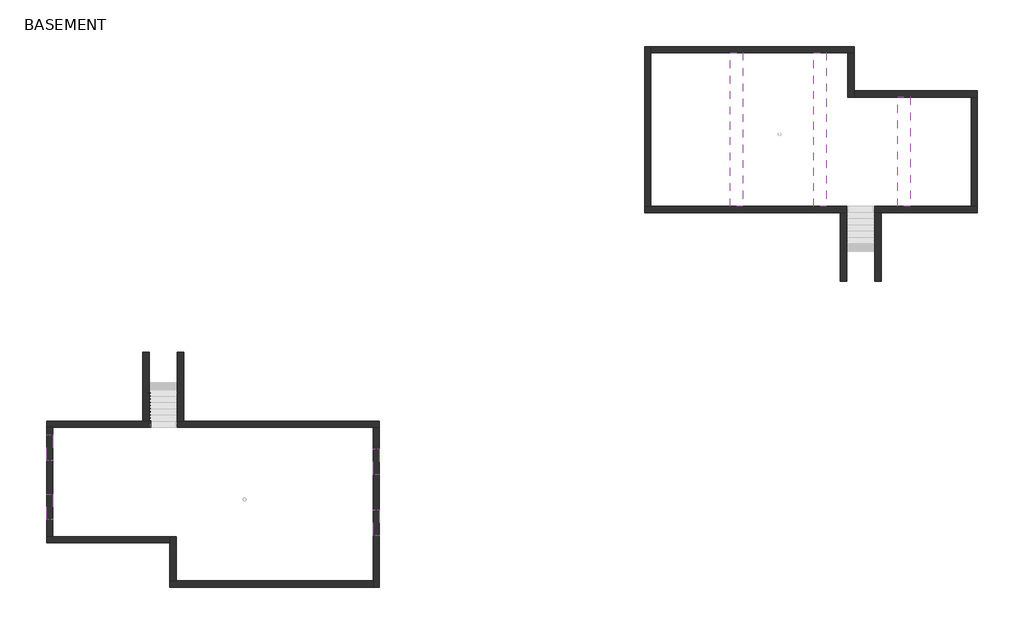
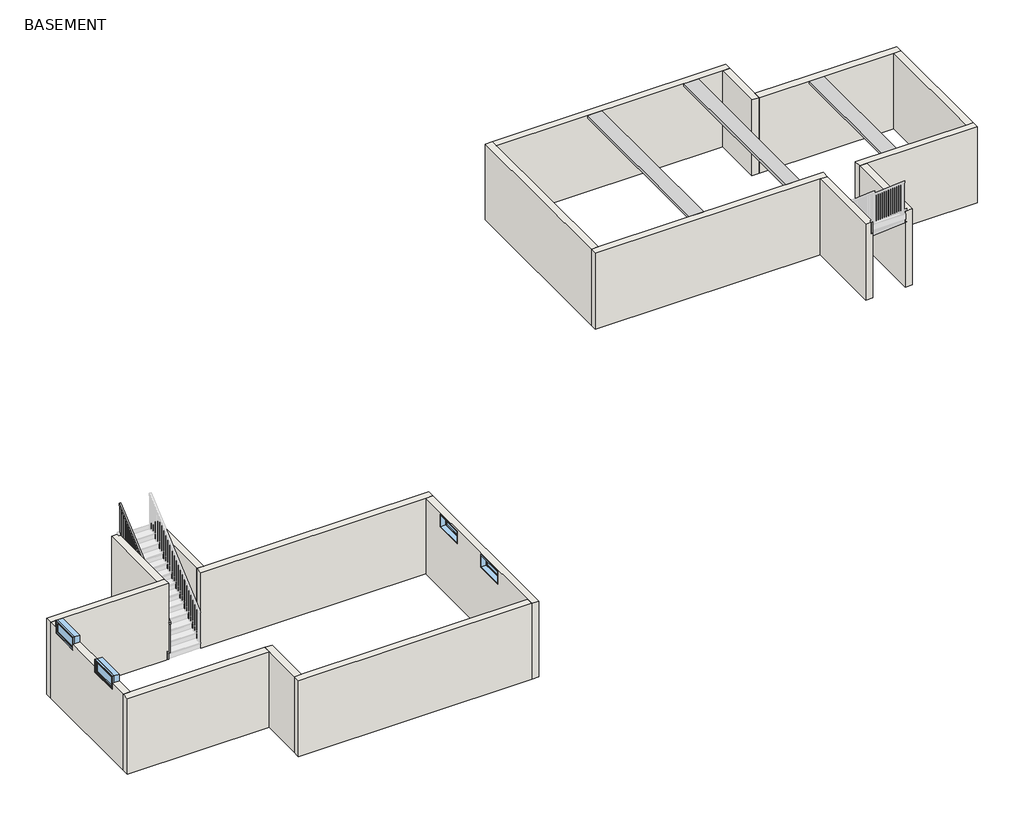
# One storey, part 1 of 2: 18 walls, 4 windows, 3 beams, 1 railing.
"""IFC4 building model written with IfcOpenShell, lengths in millimetres."""

import ifcopenshell
import ifcopenshell.guid

model = None  # the IFC model being written
_history = None  # IfcOwnerHistory: only IFC2X3 demands one
_inside = {}  # id of a spatial element -> (the spatial element, [elements in it])
_under = {}  # id of a project, library or spatial element -> (it, [spatial elements below it])
_declared = {}  # id of a project -> (the project, [libraries it declares])
_typed = {}  # id of a type object -> (the type object, [elements of that type])
_made_of = {}  # id of a material, layer set ... -> (it, [elements and type objects made of it])


def new_model(schema):
    """Start an empty IFC model of exactly this schema.

    Asked for "IFC4X3", IfcOpenShell would pick the latest addendum, in which some entities
    have other attributes; the version numbers below select the first issue.
    IFC2X3 requires an IfcOwnerHistory on every rooted entity: one is made here for all.
    """
    global model, _history
    if schema == "IFC4X3":
        model = ifcopenshell.file(schema_version=(4, 3, 0, 0))
    else:
        model = ifcopenshell.file(schema=schema)
    _inside.clear()
    _under.clear()
    _declared.clear()
    _typed.clear()
    _made_of.clear()
    _history = None
    if model.schema == "IFC2X3":
        org = make("IfcOrganization", Name="unknown")
        user = make(
            "IfcPersonAndOrganization",
            ThePerson=make("IfcPerson", FamilyName="unknown"),
            TheOrganization=org,
        )
        app = make(
            "IfcApplication",
            ApplicationDeveloper=org,
            Version="unknown",
            ApplicationFullName="unknown",
            ApplicationIdentifier="unknown",
        )
        _history = make(
            "IfcOwnerHistory",
            OwningUser=user,
            OwningApplication=app,
            ChangeAction="ADDED",
            CreationDate=0,
        )
    return model


def make(cls, **values):
    """One entity of the class cls with the attributes given. An attribute that is None is left unset."""
    return model.create_entity(
        cls, **{name: value for name, value in values.items() if value is not None}
    )


def rooted(cls, **values):
    """An entity with a GlobalId (a new one), such as an element, a storey or a relation."""
    return make(cls, GlobalId=ifcopenshell.guid.new(), OwnerHistory=_history, **values)


def si_unit(unit_type, name, prefix=None):
    """IfcSIUnit, for example si_unit("LENGTHUNIT", "METRE", prefix="MILLI")."""
    return make("IfcSIUnit", UnitType=unit_type, Prefix=prefix, Name=name)


def assignment(units):
    """IfcUnitAssignment: the units of a project."""
    return None if units is None else make("IfcUnitAssignment", Units=units)


def point(xyz):
    """IfcCartesianPoint."""
    return None if xyz is None else make("IfcCartesianPoint", Coordinates=xyz)


def direction(xyz):
    """IfcDirection."""
    return None if xyz is None else make("IfcDirection", DirectionRatios=xyz)


def frame(location, z_axis=None, x_axis=None):
    """IfcAxis2Placement3D, a coordinate frame: its origin and axes. An axis left out is left unset."""
    return make(
        "IfcAxis2Placement3D",
        Location=point(location),
        Axis=direction(z_axis),
        RefDirection=direction(x_axis),
    )


def origin():
    """The frame at (0, 0, 0) with its axes left unset."""
    return frame((0.0, 0.0, 0.0))


def place(relative_to, where):
    """IfcLocalPlacement: puts the frame where relative to a parent placement (None: the world)."""
    return make(
        "IfcLocalPlacement", PlacementRelTo=relative_to, RelativePlacement=where
    )


def context(
    kind, dimensions, precision=None, world=None, true_north=None, identifier=None
):
    """IfcGeometricRepresentationContext, for example the 3D "Model" context."""
    return make(
        "IfcGeometricRepresentationContext",
        ContextIdentifier=identifier,
        ContextType=kind,
        CoordinateSpaceDimension=dimensions,
        Precision=precision,
        WorldCoordinateSystem=world,
        TrueNorth=true_north,
    )


def project(units=None, contexts=None):
    """IfcProject with its units and contexts."""
    return rooted(
        "IfcProject",
        Name="project",
        RepresentationContexts=contexts,
        UnitsInContext=assignment(units),
    )


def spatial(cls, under=None, at=None, **own):
    """A site, building, storey or space (cls), placed at a placement, below another one or the project."""
    s = rooted(cls, ObjectPlacement=at, **own)
    if under is not None:
        _under.setdefault(under.id(), (under, []))[1].append(s)
    return s


def polyline(points):
    """IfcPolyline through the points."""
    return make("IfcPolyline", Points=[point(p) for p in points])


def outline(outer, holes=None, kind="AREA"):
    """IfcArbitraryClosedProfileDef: a profile drawn as a closed curve; with holes, ...WithVoids."""
    if holes is None:
        return make("IfcArbitraryClosedProfileDef", ProfileType=kind, OuterCurve=outer)
    return make(
        "IfcArbitraryProfileDefWithVoids",
        ProfileType=kind,
        OuterCurve=outer,
        InnerCurves=holes,
    )


def extrude(swept, where, along, depth):
    """IfcExtrudedAreaSolid: the profile swept, set in the frame where, extruded along a direction by depth."""
    return make(
        "IfcExtrudedAreaSolid",
        SweptArea=swept,
        Position=where,
        ExtrudedDirection=direction(along),
        Depth=depth,
    )


def faces_of(points, faces, orient=None, outer=None):
    """IfcFace entities. A face is a list of loops; a loop is a list of indices into points, from 0.

    orient and outer hold one flag for each loop. By default every Orientation is true, the
    first loop of a face is its IfcFaceOuterBound and the others are IfcFaceBound.
    """
    made = []
    for i, loops in enumerate(faces):
        bounds = []
        for j, loop in enumerate(loops):
            is_outer = j == 0 if outer is None else outer[i][j]
            bounds.append(
                make(
                    "IfcFaceOuterBound" if is_outer else "IfcFaceBound",
                    Bound=make("IfcPolyLoop", Polygon=[points[k] for k in loop]),
                    Orientation=True if orient is None else orient[i][j],
                )
            )
        made.append(make("IfcFace", Bounds=bounds))
    return made


def faceted_brep(points, faces, orient=None, outer=None, voids=None):
    """IfcFacetedBrep: a solid bounded by flat faces; with voids (closed shells), ...WithVoids."""
    shared = [point(p) for p in points]
    hull = make("IfcClosedShell", CfsFaces=faces_of(shared, faces, orient, outer))
    if voids is None:
        return make("IfcFacetedBrep", Outer=hull)
    return make(
        "IfcFacetedBrepWithVoids",
        Outer=hull,
        Voids=[
            make(cls, CfsFaces=faces_of(shared, fs, o, b)) for cls, fs, o, b in voids
        ],
    )


def shape(context_of_items, identifier, shape_type, items):
    """IfcShapeRepresentation: the items that make up one representation, for example the "Body"."""
    return make(
        "IfcShapeRepresentation",
        ContextOfItems=context_of_items,
        RepresentationIdentifier=identifier,
        RepresentationType=shape_type,
        Items=items,
    )


def source(mapping_origin, context_of_items, identifier, shape_type, items):
    """IfcRepresentationMap: a shape defined once, which mapped items show again and again."""
    return make(
        "IfcRepresentationMap",
        MappingOrigin=mapping_origin,
        MappedRepresentation=shape(context_of_items, identifier, shape_type, items),
    )


def transform(
    local_origin,
    x_axis=None,
    y_axis=None,
    z_axis=None,
    scale=None,
    scale2=None,
    scale3=None,
    uniform=True,
):
    """IfcCartesianTransformationOperator3D, or its non-uniform kind. x_axis, y_axis, z_axis: its Axis1, 2, 3."""
    if uniform:
        return make(
            "IfcCartesianTransformationOperator3D",
            Axis1=direction(x_axis),
            Axis2=direction(y_axis),
            LocalOrigin=point(local_origin),
            Scale=scale,
            Axis3=direction(z_axis),
        )
    return make(
        "IfcCartesianTransformationOperator3DnonUniform",
        Axis1=direction(x_axis),
        Axis2=direction(y_axis),
        LocalOrigin=point(local_origin),
        Scale=scale,
        Axis3=direction(z_axis),
        Scale2=scale2,
        Scale3=scale3,
    )


def mapped(mapping_source, mapping_target):
    """IfcMappedItem: shows the shape of a source again, moved by a transform."""
    return make(
        "IfcMappedItem", MappingSource=mapping_source, MappingTarget=mapping_target
    )


def made_of(thing, what):
    """Note that an element or type object is made of a material, layer set ...; save() writes the relation."""
    if what is not None:
        _made_of.setdefault(what.id(), (what, []))[1].append(thing)
    return thing


def element(
    cls,
    number,
    at=None,
    inside=None,
    cuts=None,
    type_object=None,
    material=None,
    context=None,
    identifier="Body",
    shape_type=None,
    held_by="IfcProductDefinitionShape",
    body=None,
    shapes=None,
    **own,
):
    """One element of the class cls, such as IfcWall. Its Tag is "e" and its number.

    at: its placement. inside: the storey or other place that contains it. cuts: it is an
    opening in that element (IfcRelVoidsElement). A single representation is given by context,
    identifier, shape_type and body (its items); several are given by shapes. held_by: the class
    of the entity that holds the representations. save() writes the other relations.
    """
    e = rooted(cls, Tag="e%d" % number, ObjectPlacement=at, **own)
    if body is not None:
        shapes = [shape(context, identifier, shape_type, body)]
    if shapes is not None:
        e.Representation = make(held_by, Representations=shapes)
    if inside is not None:
        _inside.setdefault(inside.id(), (inside, []))[1].append(e)
    if cuts is not None:
        rooted(
            "IfcRelVoidsElement", RelatingBuildingElement=cuts, RelatedOpeningElement=e
        )
    if type_object is not None:
        _typed.setdefault(type_object.id(), (type_object, []))[1].append(e)
    return made_of(e, material)


def aggregate(whole, parts):
    """IfcRelAggregates: a whole, such as a stair, and the parts it consists of."""
    return rooted("IfcRelAggregates", RelatingObject=whole, RelatedObjects=parts)


def save(model, path):
    """Write the relations noted so far, then the file.

    IfcRelAggregates (storeys below a building ...), IfcRelContainedInSpatialStructure (elements
    in a storey), IfcRelDefinesByType, IfcRelAssociatesMaterial and IfcRelDeclares: one each for
    every whole, place, type object, material and project.
    """
    for whole, parts in _under.values():
        aggregate(whole, parts)
    for where, things in _inside.values():
        rooted(
            "IfcRelContainedInSpatialStructure",
            RelatedElements=things,
            RelatingStructure=where,
        )
    for kind, things in _typed.values():
        rooted("IfcRelDefinesByType", RelatedObjects=things, RelatingType=kind)
    for what, things in _made_of.values():
        rooted("IfcRelAssociatesMaterial", RelatedObjects=things, RelatingMaterial=what)
    for by, libraries in _declared.values():
        rooted("IfcRelDeclares", RelatingContext=by, RelatedDefinitions=libraries)
    model.write(path)


def window_df5485c9(model_context):
    return source(origin(), model_context, "Body", "SweptSolid", [
        extrude(outline(polyline([(317.5, 53.975), (-393.7, 53.975), (-393.7, 66.675), (317.5, 66.675), (317.5, 53.975)])), frame((0.0, 0.0, 977.9), z_axis=(0.0, 0.0, 1.0), x_axis=(1.0, 0.0, 0.0)), (0.0, 0.0, 1.0), 254.0),
        extrude(outline(polyline([(1276.35, -438.15), (933.45, -438.15), (933.45, 361.95), (1276.35, 361.95), (1276.35, -438.15)]), holes=[polyline([(1231.9, -393.7), (1231.9, 317.5), (977.9, 317.5), (977.9, -393.7), (1231.9, -393.7)])]), frame((0.0, 38.1, 0.0), z_axis=(0.0, 1.0, 0.0), x_axis=(0.0, 0.0, 1.0)), (0.0, 0.0, 1.0), 44.45),
        extrude(outline(polyline([(1295.4, -457.2), (914.4, -457.2), (914.4, 381.0), (1295.4, 381.0), (1295.4, -457.2)]), holes=[polyline([(1263.65, -425.45), (1263.65, 349.25), (946.15, 349.25), (946.15, -425.45), (1263.65, -425.45)])]), frame((0.0, -101.6, 0.0), z_axis=(0.0, 1.0, 0.0), x_axis=(0.0, 0.0, 1.0)), (0.0, 0.0, 1.0), 139.7),
        extrude(outline(polyline([(1295.4, 381.0), (1295.4, -457.2), (914.4, -457.2), (914.4, 381.0), (1295.4, 381.0)]), holes=[polyline([(1276.35, 361.95), (933.45, 361.95), (933.45, -438.15), (1276.35, -438.15), (1276.35, 361.95)])]), frame((0.0, 38.1, 0.0), z_axis=(0.0, 1.0, 0.0), x_axis=(0.0, 0.0, 1.0)), (0.0, 0.0, 1.0), 63.5),
    ])


model = new_model("IFC4")

# Units and contexts
model_context = context("Model", 3, world=origin())
ifc_project = project(units=[si_unit("LENGTHUNIT", "METRE", prefix="MILLI")], contexts=[model_context])

# Site, building, storey
site = spatial("IfcSite", under=ifc_project)
building = spatial("IfcBuilding", under=site)
storey = spatial("IfcBuildingStorey", under=building, Name="BASEMENT", Elevation=-2266.95)

# Beams
placement = place(None, origin())
element("IfcBeam", 1, ObjectType="Concrete-Rectangular Beam : width=1' - 4\" x depth=0'  3 1/4\"", at=placement, inside=storey, context=model_context, shape_type="SweptSolid", body=[
    extrude(outline(polyline([(-3464.4595256, -410.4444564), (-3058.0595256, -410.4444564), (-3058.0595256, -5395.1944564), (-3464.4595256, -5395.1944564), (-3464.4595256, -410.4444564)])), frame((0.0, 0.0, -82.55), z_axis=(0.0, 0.0, 1.0), x_axis=(1.0, 0.0, 0.0)), (0.0, 0.0, 1.0), 82.55),
])
element("IfcBeam", 2, ObjectType="Concrete-Rectangular Beam : width=1' - 4\" x depth=0'  3 1/4\"", at=placement, inside=storey, context=model_context, shape_type="SweptSolid", body=[
    extrude(outline(polyline([(-6182.2595256, -410.4444564), (-5775.8595256, -410.4444564), (-5775.8595256, -5395.1944564), (-6182.2595256, -5395.1944564), (-6182.2595256, -410.4444564)])), frame((0.0, 0.0, -82.55), z_axis=(0.0, 0.0, 1.0), x_axis=(1.0, 0.0, 0.0)), (0.0, 0.0, 1.0), 82.55),
])
element("IfcBeam", 3, ObjectType="Concrete-Rectangular Beam : width=1' - 4\" x depth=0'  3 1/4\"", at=placement, inside=storey, context=model_context, shape_type="SweptSolid", body=[
    extrude(outline(polyline([(-746.6595256, -1845.5444564), (-340.2595256, -1845.5444564), (-340.2595256, -5395.1944564), (-746.6595256, -5395.1944564), (-746.6595256, -1845.5444564)])), frame((0.0, 0.0, -82.55), z_axis=(0.0, 0.0, 1.0), x_axis=(1.0, 0.0, 0.0)), (0.0, 0.0, 1.0), 82.55),
])

# Railing
element("IfcRailing", 4, ObjectType="Handrail - Rectangular", at=placement, inside=storey, context=model_context, shape_type="SweptSolid", body=[
    extrude(outline(polyline([(-12572.2570712, -1245.110853), (-12572.2570712, -1178.1692308), (-10133.8570712, 914.4), (-10133.8570712, 847.4583777), (-12572.2570712, -1245.110853)])), frame((-25042.4664763, 0.0, 0.0), z_axis=(1.0, 0.0, 0.0), x_axis=(0.0, 1.0, 0.0)), (0.0, 0.0, 1.0), 50.8),
    extrude(outline(polyline([(-10225.9320712, 768.4420917), (-10225.9320712, -174.3807692), (-10244.9820712, -174.3807692), (-10244.9820712, 752.0938946), (-10225.9320712, 768.4420917)])), frame((-25026.5914763, 0.0, 0.0), z_axis=(1.0, 0.0, 0.0), x_axis=(0.0, 1.0, 0.0)), (0.0, 0.0, 1.0), 19.05),
    extrude(outline(polyline([(-10327.5320712, 681.2517071), (-10327.5320712, -174.3807692), (-10346.5820712, -174.3807692), (-10346.5820712, 664.9035099), (-10327.5320712, 681.2517071)])), frame((-25026.5914763, 0.0, 0.0), z_axis=(1.0, 0.0, 0.0), x_axis=(0.0, 1.0, 0.0)), (0.0, 0.0, 1.0), 19.05),
    extrude(outline(polyline([(-10429.1320712, 594.0613224), (-10429.1320712, -348.7615385), (-10448.1820712, -348.7615385), (-10448.1820712, 577.7131253), (-10429.1320712, 594.0613224)])), frame((-25026.5914763, 0.0, 0.0), z_axis=(1.0, 0.0, 0.0), x_axis=(0.0, 1.0, 0.0)), (0.0, 0.0, 1.0), 19.05),
    extrude(outline(polyline([(-10530.7320712, 506.8709378), (-10530.7320712, -348.7615385), (-10549.7820712, -348.7615385), (-10549.7820712, 490.5227407), (-10530.7320712, 506.8709378)])), frame((-25026.5914763, 0.0, 0.0), z_axis=(1.0, 0.0, 0.0), x_axis=(0.0, 1.0, 0.0)), (0.0, 0.0, 1.0), 19.05),
    extrude(outline(polyline([(-10632.3320712, 419.6805532), (-10632.3320712, -523.1423077), (-10651.3820712, -523.1423077), (-10651.3820712, 403.3323561), (-10632.3320712, 419.6805532)])), frame((-25026.5914763, 0.0, 0.0), z_axis=(1.0, 0.0, 0.0), x_axis=(0.0, 1.0, 0.0)), (0.0, 0.0, 1.0), 19.05),
    extrude(outline(polyline([(-10733.9320712, 332.4901686), (-10733.9320712, -523.1423077), (-10752.9820712, -523.1423077), (-10752.9820712, 316.1419715), (-10733.9320712, 332.4901686)])), frame((-25026.5914763, 0.0, 0.0), z_axis=(1.0, 0.0, 0.0), x_axis=(0.0, 1.0, 0.0)), (0.0, 0.0, 1.0), 19.05),
    extrude(outline(polyline([(-10835.5320712, 245.299784), (-10835.5320712, -697.5230769), (-10854.5820712, -697.5230769), (-10854.5820712, 228.9515869), (-10835.5320712, 245.299784)])), frame((-25026.5914763, 0.0, 0.0), z_axis=(1.0, 0.0, 0.0), x_axis=(0.0, 1.0, 0.0)), (0.0, 0.0, 1.0), 19.05),
    extrude(outline(polyline([(-10937.1320712, 158.1093994), (-10937.1320712, -697.5230769), (-10956.1820712, -697.5230769), (-10956.1820712, 141.7612022), (-10937.1320712, 158.1093994)])), frame((-25026.5914763, 0.0, 0.0), z_axis=(1.0, 0.0, 0.0), x_axis=(0.0, 1.0, 0.0)), (0.0, 0.0, 1.0), 19.05),
    extrude(outline(polyline([(-11038.7320712, 70.9190147), (-11038.7320712, -871.9038462), (-11057.7820712, -871.9038462), (-11057.7820712, 54.5708176), (-11038.7320712, 70.9190147)])), frame((-25026.5914763, 0.0, 0.0), z_axis=(1.0, 0.0, 0.0), x_axis=(0.0, 1.0, 0.0)), (0.0, 0.0, 1.0), 19.05),
    extrude(outline(polyline([(-11140.3320712, -16.2713699), (-11140.3320712, -871.9038462), (-11159.3820712, -871.9038462), (-11159.3820712, -32.619567), (-11140.3320712, -16.2713699)])), frame((-25026.5914763, 0.0, 0.0), z_axis=(1.0, 0.0, 0.0), x_axis=(0.0, 1.0, 0.0)), (0.0, 0.0, 1.0), 19.05),
    extrude(outline(polyline([(-11241.9320712, -103.4617545), (-11241.9320712, -1046.2846154), (-11260.9820712, -1046.2846154), (-11260.9820712, -119.8099516), (-11241.9320712, -103.4617545)])), frame((-25026.5914763, 0.0, 0.0), z_axis=(1.0, 0.0, 0.0), x_axis=(0.0, 1.0, 0.0)), (0.0, 0.0, 1.0), 19.05),
    extrude(outline(polyline([(-11343.5320712, -190.6521391), (-11343.5320712, -1046.2846154), (-11362.5820712, -1046.2846154), (-11362.5820712, -207.0003362), (-11343.5320712, -190.6521391)])), frame((-25026.5914763, 0.0, 0.0), z_axis=(1.0, 0.0, 0.0), x_axis=(0.0, 1.0, 0.0)), (0.0, 0.0, 1.0), 19.05),
    extrude(outline(polyline([(-11445.1320712, -277.8425237), (-11445.1320712, -1220.6653846), (-11464.1820712, -1220.6653846), (-11464.1820712, -294.1907208), (-11445.1320712, -277.8425237)])), frame((-25026.5914763, 0.0, 0.0), z_axis=(1.0, 0.0, 0.0), x_axis=(0.0, 1.0, 0.0)), (0.0, 0.0, 1.0), 19.05),
    extrude(outline(polyline([(-11546.7320712, -365.0329083), (-11546.7320712, -1220.6653846), (-11565.7820712, -1220.6653846), (-11565.7820712, -381.3811054), (-11546.7320712, -365.0329083)])), frame((-25026.5914763, 0.0, 0.0), z_axis=(1.0, 0.0, 0.0), x_axis=(0.0, 1.0, 0.0)), (0.0, 0.0, 1.0), 19.05),
    extrude(outline(polyline([(-11648.3320712, -452.2232929), (-11648.3320712, -1395.0461538), (-11667.3820712, -1395.0461538), (-11667.3820712, -468.5714901), (-11648.3320712, -452.2232929)])), frame((-25026.5914763, 0.0, 0.0), z_axis=(1.0, 0.0, 0.0), x_axis=(0.0, 1.0, 0.0)), (0.0, 0.0, 1.0), 19.05),
    extrude(outline(polyline([(-11749.9320712, -539.4136776), (-11749.9320712, -1395.0461538), (-11768.9820712, -1395.0461538), (-11768.9820712, -555.7618747), (-11749.9320712, -539.4136776)])), frame((-25026.5914763, 0.0, 0.0), z_axis=(1.0, 0.0, 0.0), x_axis=(0.0, 1.0, 0.0)), (0.0, 0.0, 1.0), 19.05),
    extrude(outline(polyline([(-11851.5320712, -626.6040622), (-11851.5320712, -1569.4269231), (-11870.5820712, -1569.4269231), (-11870.5820712, -642.9522593), (-11851.5320712, -626.6040622)])), frame((-25026.5914763, 0.0, 0.0), z_axis=(1.0, 0.0, 0.0), x_axis=(0.0, 1.0, 0.0)), (0.0, 0.0, 1.0), 19.05),
    extrude(outline(polyline([(-11953.1320712, -713.7944468), (-11953.1320712, -1569.4269231), (-11972.1820712, -1569.4269231), (-11972.1820712, -730.1426439), (-11953.1320712, -713.7944468)])), frame((-25026.5914763, 0.0, 0.0), z_axis=(1.0, 0.0, 0.0), x_axis=(0.0, 1.0, 0.0)), (0.0, 0.0, 1.0), 19.05),
    extrude(outline(polyline([(-12054.7320712, -800.9848314), (-12054.7320712, -1743.8076923), (-12073.7820712, -1743.8076923), (-12073.7820712, -817.3330285), (-12054.7320712, -800.9848314)])), frame((-25026.5914763, 0.0, 0.0), z_axis=(1.0, 0.0, 0.0), x_axis=(0.0, 1.0, 0.0)), (0.0, 0.0, 1.0), 19.05),
    extrude(outline(polyline([(-12156.3320712, -888.175216), (-12156.3320712, -1743.8076923), (-12175.3820712, -1743.8076923), (-12175.3820712, -904.5234131), (-12156.3320712, -888.175216)])), frame((-25026.5914763, 0.0, 0.0), z_axis=(1.0, 0.0, 0.0), x_axis=(0.0, 1.0, 0.0)), (0.0, 0.0, 1.0), 19.05),
    extrude(outline(polyline([(-12257.9320712, -975.3656006), (-12257.9320712, -1918.1884615), (-12276.9820712, -1918.1884615), (-12276.9820712, -991.7137978), (-12257.9320712, -975.3656006)])), frame((-25026.5914763, 0.0, 0.0), z_axis=(1.0, 0.0, 0.0), x_axis=(0.0, 1.0, 0.0)), (0.0, 0.0, 1.0), 19.05),
    extrude(outline(polyline([(-12359.5320712, -1062.5559853), (-12359.5320712, -1918.1884615), (-12378.5820712, -1918.1884615), (-12378.5820712, -1078.9041824), (-12359.5320712, -1062.5559853)])), frame((-25026.5914763, 0.0, 0.0), z_axis=(1.0, 0.0, 0.0), x_axis=(0.0, 1.0, 0.0)), (0.0, 0.0, 1.0), 19.05),
    extrude(outline(polyline([(-12461.1320712, -1149.7463699), (-12461.1320712, -2092.5692308), (-12480.1820712, -2092.5692308), (-12480.1820712, -1166.094567), (-12461.1320712, -1149.7463699)])), frame((-25026.5914763, 0.0, 0.0), z_axis=(1.0, 0.0, 0.0), x_axis=(0.0, 1.0, 0.0)), (0.0, 0.0, 1.0), 19.05),
    extrude(outline(polyline([(-10133.8570712, 847.4583777), (-10133.8570712, -174.3807692), (-10152.9070712, -174.3807692), (-10152.9070712, 831.1101806), (-10133.8570712, 847.4583777)])), frame((-25026.5914763, 0.0, 0.0), z_axis=(1.0, 0.0, 0.0), x_axis=(0.0, 1.0, 0.0)), (0.0, 0.0, 1.0), 19.05),
    extrude(outline(polyline([(-12553.2070712, -1228.7626559), (-12553.2070712, -2092.5692308), (-12572.2570712, -2092.5692308), (-12572.2570712, -1245.110853), (-12553.2070712, -1228.7626559)])), frame((-25026.5914763, 0.0, 0.0), z_axis=(1.0, 0.0, 0.0), x_axis=(0.0, 1.0, 0.0)), (0.0, 0.0, 1.0), 19.05),
])

# Walls
element("IfcWall", 5, ObjectType="Generic - 8\"", at=placement, inside=storey, context=model_context, shape_type="Brep", body=[
    faceted_brep([(1844.1404744, -5395.1944564, -2266.95), (1640.9404744, -5395.1944564, -2266.95), (-1489.6095256, -5395.1944564, -2266.95), (-1489.6095256, -5395.1944564, 0.0), (1640.9404744, -5395.1944564, 0.0), (1844.1404744, -5395.1944564, 0.0), (1844.1404744, -5598.3944564, -2266.95), (1844.1404744, -5598.3944564, 0.0), (-1286.4095256, -5598.3944564, 0.0), (-1489.6095256, -5598.3944564, 0.0), (-1489.6095256, -5598.3944564, -2266.95), (-1286.4095256, -5598.3944564, -2266.95)], [[[0, 1, 2, 3, 4, 5]], [[6, 7, 8, 9, 10, 11]], [[2, 1, 0, 6, 11, 10]], [[5, 4, 3, 9, 8, 7]], [[0, 5, 7, 6]], [[3, 2, 10, 9]]]),
])
element("IfcWall", 6, ObjectType="Generic - 8\"", at=placement, inside=storey, context=model_context, shape_type="Brep", body=[
    faceted_brep([(-8760.3595256, -5395.1944564, -2266.95), (-8760.3595256, -410.4444564, -2266.95), (-8760.3595256, -207.2444564, -2266.95), (-8760.3595256, -207.2444564, 0.0), (-8760.3595256, -410.4444564, 0.0), (-8760.3595256, -5395.1944564, 0.0), (-8963.5595256, -5395.1944564, -2266.95), (-8963.5595256, -5395.1944564, 0.0), (-8963.5595256, -207.2444564, 0.0), (-8963.5595256, -207.2444564, -2266.95)], [[[0, 1, 2, 3, 4, 5]], [[6, 7, 8, 9]], [[2, 1, 0, 6, 9]], [[5, 4, 3, 8, 7]], [[0, 5, 7, 6]], [[3, 2, 9, 8]]]),
])
element("IfcWall", 7, ObjectType="Generic - 8\"", at=placement, inside=storey, context=model_context, shape_type="Brep", body=[
    faceted_brep([(-8760.3595256, -410.4444564, -2266.95), (-2365.9095256, -410.4444564, -2266.95), (-2162.7095256, -410.4444564, -2266.95), (-2162.7095256, -410.4444564, 0.0), (-2365.9095256, -410.4444564, 0.0), (-8760.3595256, -410.4444564, 0.0), (-8760.3595256, -207.2444564, -2266.95), (-8760.3595256, -207.2444564, 0.0), (-2162.7095256, -207.2444564, 0.0), (-2162.7095256, -207.2444564, -2266.95)], [[[0, 1, 2, 3, 4, 5]], [[6, 7, 8, 9]], [[2, 1, 0, 6, 9]], [[5, 4, 3, 8, 7]], [[0, 5, 7, 6]], [[3, 2, 9, 8]]]),
])
element("IfcWall", 8, ObjectType="Generic - 8\"", at=placement, inside=storey, context=model_context, shape_type="Brep", body=[
    faceted_brep([(-2365.9095256, -410.4444564, -2266.95), (-2365.9095256, -1845.5444564, -2266.95), (-2365.9095256, -1845.5444564, 0.0), (-2365.9095256, -410.4444564, 0.0), (-2162.7095256, -410.4444564, -2266.95), (-2162.7095256, -410.4444564, 0.0), (-2162.7095256, -1642.3444564, 0.0), (-2162.7095256, -1845.5444564, 0.0), (-2162.7095256, -1845.5444564, -2266.95), (-2162.7095256, -1642.3444564, -2266.95)], [[[0, 1, 2, 3]], [[4, 5, 6, 7, 8, 9]], [[1, 0, 4, 9, 8]], [[3, 2, 7, 6, 5]], [[0, 3, 5, 4]], [[2, 1, 8, 7]]]),
])
element("IfcWall", 9, ObjectType="Generic - 8\"", at=placement, inside=storey, context=model_context, shape_type="Brep", body=[
    faceted_brep([(-2162.7095256, -1845.5444564, -2266.95), (1640.9404744, -1845.5444564, -2266.95), (1844.1404744, -1845.5444564, -2266.95), (1844.1404744, -1845.5444564, 0.0), (1640.9404744, -1845.5444564, 0.0), (-2162.7095256, -1845.5444564, 0.0), (-2162.7095256, -1642.3444564, -2266.95), (-2162.7095256, -1642.3444564, 0.0), (1844.1404744, -1642.3444564, 0.0), (1844.1404744, -1642.3444564, -2266.95)], [[[0, 1, 2, 3, 4, 5]], [[6, 7, 8, 9]], [[2, 1, 0, 6, 9]], [[5, 4, 3, 8, 7]], [[0, 5, 7, 6]], [[3, 2, 9, 8]]]),
])
element("IfcWall", 10, ObjectType="Generic - 8\"", at=placement, inside=storey, context=model_context, shape_type="SweptSolid", body=[
    extrude(outline(polyline([(1640.9404744, -5395.1944564), (1640.9404744, -1845.5444564), (1844.1404744, -1845.5444564), (1844.1404744, -5395.1944564), (1640.9404744, -5395.1944564)])), frame((0.0, 0.0, -2266.95), z_axis=(0.0, 0.0, 1.0), x_axis=(1.0, 0.0, 0.0)), (0.0, 0.0, 1.0), 2266.95),
])
element("IfcWall", 11, ObjectType="Generic - 8\"", at=placement, inside=storey, context=model_context, shape_type="Brep", body=[
    faceted_brep([(-2404.0095256, -5395.1944564, -2266.95), (-8760.3595256, -5395.1944564, -2266.95), (-8963.5595256, -5395.1944564, -2266.95), (-8963.5595256, -5395.1944564, 0.0), (-8760.3595256, -5395.1944564, 0.0), (-2404.0095256, -5395.1944564, 0.0), (-2404.0095256, -5598.3944564, -2266.95), (-2404.0095256, -5598.3944564, 0.0), (-2607.2095256, -5598.3944564, 0.0), (-8963.5595256, -5598.3944564, 0.0), (-8963.5595256, -5598.3944564, -2266.95), (-2607.2095256, -5598.3944564, -2266.95)], [[[0, 1, 2, 3, 4, 5]], [[6, 7, 8, 9, 10, 11]], [[2, 1, 0, 6, 11, 10]], [[5, 4, 3, 9, 8, 7]], [[3, 2, 10, 9]], [[0, 5, 7, 6]]]),
])
element("IfcWall", 12, ObjectType="Generic - 8\"", at=placement, inside=storey, context=model_context, shape_type="SweptSolid", body=[
    extrude(outline(polyline([(-1489.6095256, -7833.5944564), (-1489.6095256, -5598.3944564), (-1286.4095256, -5598.3944564), (-1286.4095256, -7833.5944564), (-1489.6095256, -7833.5944564)])), frame((0.0, 0.0, -2266.95), z_axis=(0.0, 0.0, 1.0), x_axis=(1.0, 0.0, 0.0)), (0.0, 0.0, 1.0), 2266.95),
])
element("IfcWall", 13, ObjectType="Generic - 8\"", at=placement, inside=storey, context=model_context, shape_type="SweptSolid", body=[
    extrude(outline(polyline([(-2404.0095256, -5598.3944564), (-2404.0095256, -7833.5944564), (-2607.2095256, -7833.5944564), (-2607.2095256, -5598.3944564), (-2404.0095256, -5598.3944564)])), frame((0.0, 0.0, -2266.95), z_axis=(0.0, 0.0, 1.0), x_axis=(1.0, 0.0, 0.0)), (0.0, 0.0, 1.0), 2266.95),
])
element("IfcWall", 14, ObjectType="Generic - 8\"", at=placement, inside=storey, context=model_context, shape_type="Brep", body=[
    faceted_brep([(-28382.5664763, -12572.2570712, -2266.95), (-28179.3664763, -12572.2570712, -2266.95), (-25048.8164763, -12572.2570712, -2266.95), (-25048.8164763, -12572.2570712, 0.0), (-28179.3664763, -12572.2570712, 0.0), (-28382.5664763, -12572.2570712, 0.0), (-28382.5664763, -12369.0570712, -2266.95), (-28382.5664763, -12369.0570712, 0.0), (-25252.0164763, -12369.0570712, 0.0), (-25048.8164763, -12369.0570712, 0.0), (-25048.8164763, -12369.0570712, -2266.95), (-25252.0164763, -12369.0570712, -2266.95)], [[[0, 1, 2, 3, 4, 5]], [[6, 7, 8, 9, 10, 11]], [[2, 1, 0, 6, 11, 10]], [[5, 4, 3, 9, 8, 7]], [[0, 5, 7, 6]], [[3, 2, 10, 9]]]),
])
element("IfcWall", 15, ObjectType="Generic - 8\"", at=placement, inside=storey, context=model_context, shape_type="Brep", body=[
    faceted_brep([(-17778.0664763, -12572.2570712, -2266.95), (-17778.0664763, -17557.0070712, -2266.95), (-17778.0664763, -17760.2070712, -2266.95), (-17778.0664763, -17760.2070712, 0.0), (-17778.0664763, -17557.0070712, 0.0), (-17778.0664763, -12572.2570712, 0.0), (-17778.0664763, -14108.9570712, -57.15), (-17778.0664763, -14108.9570712, -438.15), (-17778.0664763, -13270.7570712, -438.15), (-17778.0664763, -13270.7570712, -57.15), (-17778.0664763, -16093.3320712, -57.15), (-17778.0664763, -16093.3320712, -438.15), (-17778.0664763, -15255.1320712, -438.15), (-17778.0664763, -15255.1320712, -57.15), (-17574.8664763, -12572.2570712, -2266.95), (-17574.8664763, -12572.2570712, 0.0), (-17574.8664763, -17760.2070712, 0.0), (-17574.8664763, -17760.2070712, -2266.95), (-17574.8664763, -14108.9570712, -57.15), (-17574.8664763, -13270.7570712, -57.15), (-17574.8664763, -13270.7570712, -438.15), (-17574.8664763, -14108.9570712, -438.15), (-17574.8664763, -16093.3320712, -57.15), (-17574.8664763, -15255.1320712, -57.15), (-17574.8664763, -15255.1320712, -438.15), (-17574.8664763, -16093.3320712, -438.15)], [[[0, 1, 2, 3, 4, 5], [6, 7, 8, 9], [10, 11, 12, 13]], [[14, 15, 16, 17], [18, 19, 20, 21], [22, 23, 24, 25]], [[2, 1, 0, 14, 17]], [[5, 4, 3, 16, 15]], [[0, 5, 15, 14]], [[3, 2, 17, 16]], [[7, 6, 18, 21]], [[8, 7, 21, 20]], [[9, 8, 20, 19]], [[6, 9, 19, 18]], [[11, 10, 22, 25]], [[12, 11, 25, 24]], [[13, 12, 24, 23]], [[10, 13, 23, 22]]]),
])
element("IfcWall", 16, ObjectType="Generic - 8\"", at=placement, inside=storey, context=model_context, shape_type="Brep", body=[
    faceted_brep([(-17778.0664763, -17557.0070712, -2266.95), (-24172.5164763, -17557.0070712, -2266.95), (-24375.7164763, -17557.0070712, -2266.95), (-24375.7164763, -17557.0070712, 0.0), (-24172.5164763, -17557.0070712, 0.0), (-17778.0664763, -17557.0070712, 0.0), (-17778.0664763, -17760.2070712, -2266.95), (-17778.0664763, -17760.2070712, 0.0), (-24375.7164763, -17760.2070712, 0.0), (-24375.7164763, -17760.2070712, -2266.95)], [[[0, 1, 2, 3, 4, 5]], [[6, 7, 8, 9]], [[2, 1, 0, 6, 9]], [[5, 4, 3, 8, 7]], [[0, 5, 7, 6]], [[3, 2, 9, 8]]]),
])
element("IfcWall", 17, ObjectType="Generic - 8\"", at=placement, inside=storey, context=model_context, shape_type="Brep", body=[
    faceted_brep([(-24172.5164763, -17557.0070712, -2266.95), (-24172.5164763, -16121.9070712, -2266.95), (-24172.5164763, -16121.9070712, 0.0), (-24172.5164763, -17557.0070712, 0.0), (-24375.7164763, -17557.0070712, -2266.95), (-24375.7164763, -17557.0070712, 0.0), (-24375.7164763, -16325.1070712, 0.0), (-24375.7164763, -16121.9070712, 0.0), (-24375.7164763, -16121.9070712, -2266.95), (-24375.7164763, -16325.1070712, -2266.95)], [[[0, 1, 2, 3]], [[4, 5, 6, 7, 8, 9]], [[1, 0, 4, 9, 8]], [[3, 2, 7, 6, 5]], [[0, 3, 5, 4]], [[2, 1, 8, 7]]]),
])
element("IfcWall", 18, ObjectType="Generic - 8\"", at=placement, inside=storey, context=model_context, shape_type="Brep", body=[
    faceted_brep([(-24375.7164763, -16121.9070712, -2266.95), (-28179.3664763, -16121.9070712, -2266.95), (-28382.5664763, -16121.9070712, -2266.95), (-28382.5664763, -16121.9070712, 0.0), (-28179.3664763, -16121.9070712, 0.0), (-24375.7164763, -16121.9070712, 0.0), (-24375.7164763, -16325.1070712, -2266.95), (-24375.7164763, -16325.1070712, 0.0), (-28382.5664763, -16325.1070712, 0.0), (-28382.5664763, -16325.1070712, -2266.95)], [[[0, 1, 2, 3, 4, 5]], [[6, 7, 8, 9]], [[2, 1, 0, 6, 9]], [[5, 4, 3, 8, 7]], [[0, 5, 7, 6]], [[3, 2, 9, 8]]]),
])
element("IfcWall", 19, ObjectType="Generic - 8\"", at=placement, inside=storey, context=model_context, shape_type="SweptSolid", body=[
    extrude(outline(polyline([(-12572.2570712, -2266.95), (-16121.9070712, -2266.95), (-16121.9070712, 0.0), (-15575.8070712, 0.0), (-15575.8070712, -177.7746), (-14737.6070712, -177.7746), (-14737.6070712, 0.0), (-13651.7570712, 0.0), (-13651.7570712, -177.7746), (-12813.5570712, -177.7746), (-12813.5570712, 0.0), (-12572.2570712, 0.0), (-12572.2570712, -2266.95)])), frame((-28382.5664763, 0.0, 0.0), z_axis=(1.0, 0.0, 0.0), x_axis=(0.0, 1.0, 0.0)), (0.0, 0.0, 1.0), 203.2),
])
element("IfcWall", 20, ObjectType="Generic - 8\"", at=placement, inside=storey, context=model_context, shape_type="Brep", body=[
    faceted_brep([(-24134.4164763, -12572.2570712, -2266.95), (-17778.0664763, -12572.2570712, -2266.95), (-17574.8664763, -12572.2570712, -2266.95), (-17574.8664763, -12572.2570712, 0.0), (-17778.0664763, -12572.2570712, 0.0), (-24134.4164763, -12572.2570712, 0.0), (-24134.4164763, -12369.0570712, -2266.95), (-24134.4164763, -12369.0570712, 0.0), (-23931.2164763, -12369.0570712, 0.0), (-17574.8664763, -12369.0570712, 0.0), (-17574.8664763, -12369.0570712, -2266.95), (-23931.2164763, -12369.0570712, -2266.95)], [[[0, 1, 2, 3, 4, 5]], [[6, 7, 8, 9, 10, 11]], [[2, 1, 0, 6, 11, 10]], [[5, 4, 3, 9, 8, 7]], [[3, 2, 10, 9]], [[0, 5, 7, 6]]]),
])
element("IfcWall", 21, ObjectType="Generic - 8\"", at=placement, inside=storey, context=model_context, shape_type="SweptSolid", body=[
    extrude(outline(polyline([(-25048.8164763, -10133.8570712), (-25048.8164763, -12369.0570712), (-25252.0164763, -12369.0570712), (-25252.0164763, -10133.8570712), (-25048.8164763, -10133.8570712)])), frame((0.0, 0.0, -2266.95), z_axis=(0.0, 0.0, 1.0), x_axis=(1.0, 0.0, 0.0)), (0.0, 0.0, 1.0), 2266.95),
])
element("IfcWall", 22, ObjectType="Generic - 8\"", at=placement, inside=storey, context=model_context, shape_type="SweptSolid", body=[
    extrude(outline(polyline([(-24134.4164763, -12369.0570712), (-24134.4164763, -10133.8570712), (-23931.2164763, -10133.8570712), (-23931.2164763, -12369.0570712), (-24134.4164763, -12369.0570712)])), frame((0.0, 0.0, -2266.95), z_axis=(0.0, 0.0, 1.0), x_axis=(1.0, 0.0, 0.0)), (0.0, 0.0, 1.0), 2266.95),
])

# Windows
window_shape = window_df5485c9(model_context)
element("IfcWindow", 23, ObjectType="Fixed : 2'-9\" x 1'-3\"", at=placement, inside=storey, context=model_context, shape_type="MappedRepresentation", body=[
    mapped(window_shape, transform((-28280.9664763, -15118.6070712, -1092.1746), x_axis=(0.0, 1.0, 0.0), y_axis=(-1.0, 0.0, 0.0), z_axis=(0.0, 0.0, 1.0))),
])
element("IfcWindow", 24, ObjectType="Fixed : 2'-9\" x 1'-3\"", at=placement, inside=storey, context=model_context, shape_type="MappedRepresentation", body=[
    mapped(window_shape, transform((-28280.9664763, -13194.5570712, -1092.1746), x_axis=(0.0, 1.0, 0.0), y_axis=(-1.0, 0.0, 0.0), z_axis=(0.0, 0.0, 1.0))),
])
element("IfcWindow", 25, ObjectType="Fixed : 2'-9\" x 1'-3\"", at=placement, inside=storey, context=model_context, shape_type="MappedRepresentation", body=[
    mapped(window_shape, transform((-17676.4664763, -13727.9570712, -1352.55), x_axis=(0.0, -1.0, 0.0), y_axis=(1.0, 0.0, 0.0), z_axis=(0.0, 0.0, 1.0))),
])
element("IfcWindow", 26, ObjectType="Fixed : 2'-9\" x 1'-3\"", at=placement, inside=storey, context=model_context, shape_type="MappedRepresentation", body=[
    mapped(window_shape, transform((-17676.4664763, -15712.3320712, -1352.55), x_axis=(0.0, -1.0, 0.0), y_axis=(1.0, 0.0, 0.0), z_axis=(0.0, 0.0, 1.0))),
])

save(model, "model.ifc")

# Revit data of these elements
# Project information
#   Project Issue Date = "Issue Date"
#   Project Status = "Project Status"
#   Client Name = "Owner"
#   Project Address = "Enter address here"
#   Project Name = "Project Name"
#   Project Number = "Project Number"
# Grids (mm)
#   "B": line (-20559.366, -20036.147) -> (-20559.366, -11545.141)
#   "C": line (-23277.166, -20036.147) -> (-23277.166, -11545.141)
#   "D": line (-25994.966, -20036.147) -> (-25994.966, -11545.141)
#   "1": line (-5979.06, 2068.696) -> (-5979.06, -6422.311)
#   "2": line (-3261.26, 2068.696) -> (-3261.26, -6422.311)
#   "3": line (-543.46, 2068.696) -> (-543.46, -6422.311)
# Type "Concrete-Rectangular Beam : width=1' - 4\" x depth=0'  3 1/4\""
#   Assembly Code = "B10"
#   Length [instance default] = 5' - 0"
#   b = 1' - 4"
#   h = 0' - 3 1/4"
#   Structural Material [instance default] = Concrete, Cast-in-Place gray
# Type "Handrail - Rectangular"
#   Assembly Code = "C2010400"
#   built-in parameter 1008612 = 0.0416667 (stored number, unit not read)
#   built-in parameter 1008611 = 0.0416667 (stored number, unit not read)
#   built-in parameter 1008609 = 0.333333 (stored number, unit not read)
#   built-in parameter 1008604 = 0.166667 (stored number, unit not read)
#   built-in parameter 1008603 = 0.166667 (stored number, unit not read)
#   Railing Height = 3' - 0"
#   built-in parameter 1008630 = 2
#   built-in parameter 1008610 = 2
#   built-in parameter 1008618 = Baluster - Square : 3/4"
# Type "Generic - 8\""
#   Assembly Code = "B2010"
#   Layers, outside or top first: 0' - 8" no material (function 1)
# Type "Fixed : 2'-9\" x 1'-3\""
#   Type Mark = "29"
#   Construction Type Id = "GSP4R"
#   Assembly Code = "B2020100"
#   Analytic Construction = "1/8 in Pilkington single glazing"
#   Visual Light Transmittance = 0.9
#   Solar Heat Gain Coefficient = 0.78
#   Heat Transfer Coefficient (U) = 3.6886 W/(m²·K)
#   Height = 1' - 3"
#   Default Sill Height = 3' - 0"
#   Width = 2' - 9"
#   Window Inset = 0' - 0 3/4"
#   Glass Pane Material = Glass
#   Sash Material = Sash
#   Wall Closure = (empty or 0)
# Element 1 (IfcBeam, "Concrete-Rectangular Beam : width=1' - 4\" x depth=0'  3 1/4\"")
#   Structural Material = Concrete, Cast-in-Place gray
#   Phase Created = New Construction
#   Materials on its faces: "Concrete, Cast-in-Place gray"
# Elements 2, 3 (IfcBeam, "Concrete-Rectangular Beam : width=1' - 4\" x depth=0'  3 1/4\"")
#   Comments = ""
#   Structural Material = Concrete, Cast-in-Place gray
#   Phase Created = New Construction
#   Materials on its faces: "Concrete, Cast-in-Place gray"
# Element 4 (IfcRailing, "Handrail - Rectangular")
#   Phase Created = New Construction
# Elements 5, 6, 7, 8, 9, 10, 11, 12, 13, 14, 15, 16, 17, 18, 19, 20, 21, 22 (IfcWall, "Generic - 8\"")
#   Top Offset = 0' - 0"
#   Base Offset = 0' - 0"
#   wall height = 7' - 5 1/4"
#   Phase Created = New Construction
#   Base Constraint = BASEMENT
#   Top Constraint = LEVEL 1
#   Materials on its faces: "Default Wall"
# Element 23 (IfcWindow, "Fixed : 2'-9\" x 1'-3\"")
#   Mark = "26"
#   Phase Created = New Construction
#   Materials on its faces: "Sash", "Glass"
# Element 24 (IfcWindow, "Fixed : 2'-9\" x 1'-3\"")
#   Mark = "27"
#   Phase Created = New Construction
#   Materials on its faces: "Sash", "Glass"
# Element 25 (IfcWindow, "Fixed : 2'-9\" x 1'-3\"")
#   Mark = "28"
#   Phase Created = New Construction
#   Materials on its faces: "Sash", "Glass"
# Element 26 (IfcWindow, "Fixed : 2'-9\" x 1'-3\"")
#   Mark = "29"
#   Phase Created = New Construction
#   Materials on its faces: "Sash", "Glass"
# Materials
#   "Concrete, Cast-in-Place gray": class "Concrete", colour RGB 192 192 192, transparency 0, Description = "Cast-in-place concrete", Cost = 0
#   "Glass": class "Glass", colour RGB 0 128 192, transparency 0.75, Description = "Soda Lime Glass", Cost = 0
#   "Sash": class "Wood", colour RGB 224 178 126, transparency 0, Cost = 0
#   "Default Wall": class "Miscellaneous", colour RGB 128 128 128, transparency 0, Cost = 0
